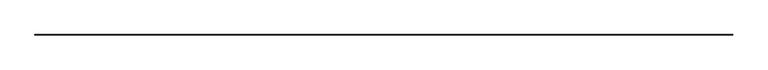
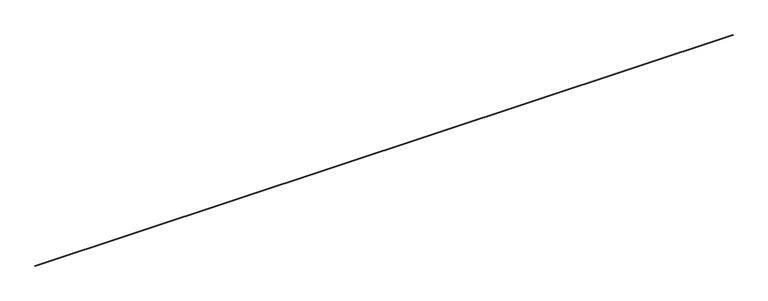
"""IFC4 building model written with IfcOpenShell, lengths in millimetres: proxy geometry, Inner panel:Inner panel:1:Inner panel:1 : Inner panel:Inner panel:300324:2:Inner panel:1:Inner panel:1 : Inner panel:Inner panel:300324:2 : Inner panel:Inner panel:1:Inner panel:1 : Inner panel:Inner panel:300324:300043:41 : Inner panel:Inner panel:1:Inner panel:1 : Inner panel:Inner panel:300324:2:Inner panel:1:Inner panel:1 : Inner panel:Inner panel:300324:2 : Inner panel:Inner panel:1:Inner panel:1 : Inner panel:Inner panel:300324:300043:308120."""

from ifc_helpers import new_model, si_unit, frame, origin, place, context, project, spatial, polyline, outline, extrude, source, transform, mapped, element, save


def generic_models_609fcc24(model_context):
    return source(origin(), model_context, "Body", "SweptSolid", [
        extrude(outline(polyline([(-579794.9881607, 3878.6695938), (-579796.5742845, 3916.7365639), (-579758.5073144, 3918.3226877), (-579756.9211906, 3880.2557176), (-579794.9881607, 3878.6695938)]), holes=[polyline([(-579792.7081078, 3881.1479122), (-579759.399509, 3882.5357705), (-579760.7873673, 3915.8443693), (-579794.0959661, 3914.456511), (-579792.7081078, 3881.1479122)])]), frame((579104.5117239, 0.0, 0.0), z_axis=(1.0, 0.0, 0.0), x_axis=(0.0, 1.0, 0.0)), (0.0, 0.0, 1.0), 88442.8),
    ])


if __name__ == "__main__":
    model = new_model("IFC4")
    model_context = context("Model", 3, world=origin())
    ifc_project = project(units=[si_unit("LENGTHUNIT", "METRE", prefix="MILLI")], contexts=[model_context])
    site = spatial("IfcSite", under=ifc_project)
    building = spatial("IfcBuilding", under=site)
    placement = place(None, origin())
    generic_models_shape = generic_models_609fcc24(model_context)
    element("IfcBuildingElementProxy", 1, Name="Inner panel:Inner panel:1:Inner panel:1 : Inner panel:Inner panel:300324:2:Inner panel:1:Inner panel:1 : Inner panel:Inner panel:300324:2 : Inner panel:Inner panel:1:Inner panel:1 : Inner panel:Inner panel:300324:300043:41 : Inner panel:Inner panel:1:Inner panel:1 : Inner panel:Inner panel:300324:2:Inner panel:1:Inner panel:1 : Inner panel:Inner panel:300324:2 : Inner panel:Inner panel:1:Inner panel:1 : Inner panel:Inner panel:300324:300043:308120", ObjectType="Inner panel:Inner panel:1:Inner panel:1 : Inner panel:Inner panel:300324:2:Inner panel:1:Inner panel:1 : Inner panel:Inner panel:300324:2 : Inner panel:Inner panel:1:Inner panel:1 : Inner panel:Inner panel:300324:300043:41 : Inner panel:Inner panel:1:Inner panel:1 : Inner panel:Inner panel:300324:2:Inner panel:1:Inner panel:1 : Inner panel:Inner panel:300324:2 : Inner panel:Inner panel:1:Inner panel:1 : Inner panel:Inner panel:300324:300043:308120", at=placement, inside=building, context=model_context, shape_type="MappedRepresentation", body=[
        mapped(generic_models_shape, transform((0.0, 0.0, 0.0), x_axis=(1.0, 0.0, 0.0), y_axis=(0.0, 1.0, 0.0), z_axis=(0.0, 0.0, 1.0))),
    ])
    save(model, "model.ifc")

# Revit data of these elements
# Type "Inner panel:Inner panel:1:Inner panel:1 : Inner panel:Inner panel:300324:2:Inner panel:1:Inner panel:1 : Inner panel:Inner panel:300324:2 : Inner panel:Inner panel:1:Inner panel:1 : Inner panel:Inner panel:300324:300043:41 : Inner panel:Inner panel:1:Inner panel:1 : Inner panel:Inner panel:300324:2:Inner panel:1:Inner panel:1 : Inner panel:Inner panel:300324:2 : Inner panel:Inner panel:1:Inner panel:1 : Inner panel:Inner panel:300324:300043:308120"
#   NameOverride = "Inner panel:Inner panel:1:Inner panel:1 : Inner panel:Inner panel:300324:2:Inner panel:1:Inner panel:1 : Inner panel:Inner panel:300324:2 : Inner panel:Inner panel:1:Inner panel:1 : Inner panel:Inner panel:300324:300043:308120"
#   ObjectTypeOverride = "Inner panel:1:Inner panel:1 : Inner panel:Inner panel:300324:2 : Inner panel:Inner panel:1:Inner panel:1 : Inner panel:Inner panel:300324:300043"
#   Reference = "Inner panel"
#   Tag = "308120"
# Element 1 (IfcBuildingElementProxy, "Inner panel:Inner panel:1:Inner panel:1 : Inner panel:Inner panel:300324:2:Inner panel:1:Inner panel:1 : Inner panel:Inner panel:300324:2 : Inner panel:Inner panel:1:Inner panel:1 : Inner panel:Inner panel:300324:300043:41 : Inner panel:Inner panel:1:Inner panel:1 : Inner panel:Inner panel:300324:2:Inner panel:1:Inner panel:1 : Inner panel:Inner panel:300324:2 : Inner panel:Inner panel:1:Inner panel:1 : Inner panel:Inner panel:300324:300043:308120")
#   Materials on its faces: "1 1/2\" X 1 1/2\" x 1/8\" ALUM. TUBE (6061-T6) - (2) #16 WOOD SCREWS WITH 2.5\" EMBED AT EACH GLULAM - (1) SCREW AT ENDS"
# Materials
#   "1 1/2\" X 1 1/2\" x 1/8\" ALUM. TUBE (6061-T6) - (2) #16 WOOD SCREWS WITH 2.5\" EMBED AT EACH GLULAM - (1) SCREW AT ENDS": class "Unassigned", colour RGB 202 201 200, transparency 0, Cost = 0
